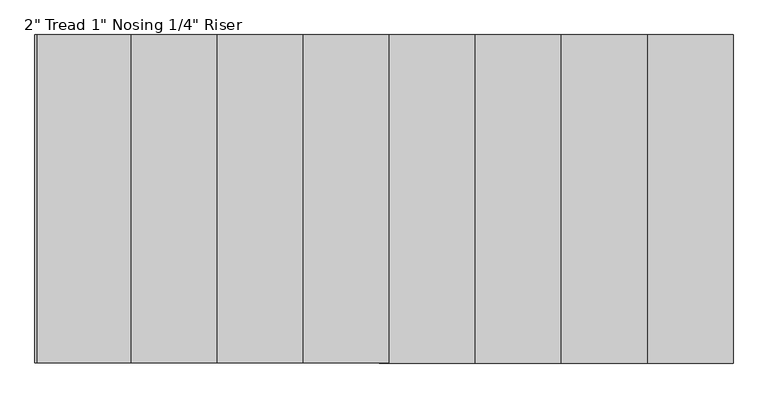
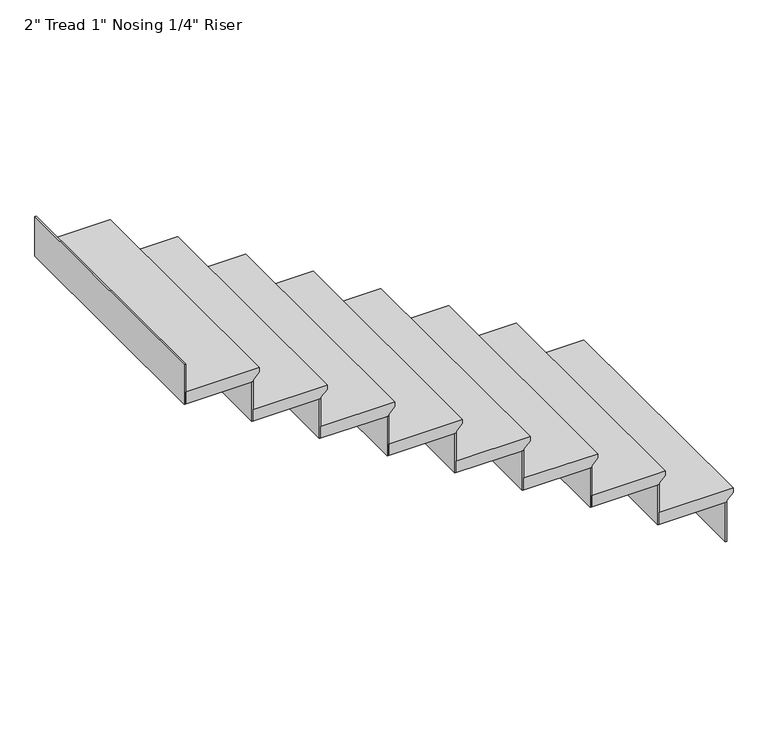
"""IFC4 building model written with IfcOpenShell, lengths in millimetres: stair flight geometry."""

from ifc_helpers import new_model, si_unit, origin, place, context, project, spatial, faceted_brep, source, transform, mapped, element, save


def stair_flight_205345c0(model_context):
    return source(origin(), model_context, "Body", "Brep", [
        faceted_brep([(665956.388677, -549416.0413841, 1710.8959459), (665956.388677, -549416.0413841, 1729.9459459), (665956.388677, -550482.8413841, 1729.9459459), (665956.388677, -550482.8413841, 1710.8959459), (665930.988677, -549416.0413841, 1685.4959459), (665930.988677, -550482.8413841, 1685.4959459), (665651.588677, -549416.0413841, 1729.9459459), (665651.588677, -550482.8413841, 1729.9459459), (665930.988677, -550482.8413841, 1679.1459459), (665651.588677, -550482.8413841, 1679.1459459), (665651.588677, -549416.0413841, 1679.1459459), (665930.988677, -549416.0413841, 1679.1459459)], [[[0, 1, 2, 3]], [[4, 0, 3, 5]], [[2, 1, 6, 7]], [[8, 9, 10, 11]], [[2, 7, 9, 8, 5, 3]], [[8, 11, 4, 5]], [[6, 1, 0, 4, 11, 10]], [[7, 6, 10, 9]]]),
        faceted_brep([(665930.988677, -549416.0413841, 1679.1459459), (665930.988677, -549416.0413841, 1506.1513514), (665924.638677, -549416.0413841, 1506.1513514), (665924.638677, -549416.0413841, 1679.1459459), (665930.988677, -550482.8413841, 1679.1459459), (665924.638677, -550482.8413841, 1679.1459459), (665924.638677, -550482.8413841, 1506.1513514), (665930.988677, -550482.8413841, 1506.1513514)], [[[0, 1, 2, 3]], [[4, 5, 6, 7]], [[1, 0, 4, 7]], [[2, 1, 7, 6]], [[3, 2, 6, 5]], [[0, 3, 5, 4]]]),
        faceted_brep([(665651.588677, -549416.0413841, 1852.1405405), (665651.588677, -549416.0413841, 1679.1459459), (665645.238677, -549416.0413841, 1679.1459459), (665645.238677, -549416.0413841, 1852.1405405), (665651.588677, -550482.8413841, 1852.1405405), (665645.238677, -550482.8413841, 1852.1405405), (665645.238677, -550482.8413841, 1679.1459459), (665651.588677, -550482.8413841, 1679.1459459)], [[[0, 1, 2, 3]], [[4, 5, 6, 7]], [[1, 0, 4, 7]], [[2, 1, 7, 6]], [[3, 2, 6, 5]], [[0, 3, 5, 4]]]),
        faceted_brep([(665676.988677, -550482.8413841, 1902.9405405), (665676.988677, -549416.0413841, 1902.9405405), (665372.188677, -549416.0413841, 1902.9405405), (665372.188677, -550482.8413841, 1902.9405405), (665651.588677, -550482.8413841, 1852.1405405), (665372.188677, -550482.8413841, 1852.1405405), (665372.188677, -549416.0413841, 1852.1405405), (665651.588677, -549416.0413841, 1852.1405405), (665651.588677, -550482.8413841, 1858.4905405), (665676.988677, -550482.8413841, 1883.8905405), (665651.588677, -549416.0413841, 1858.4905405), (665676.988677, -549416.0413841, 1883.8905405)], [[[0, 1, 2, 3]], [[4, 5, 6, 7]], [[0, 3, 5, 4, 8, 9]], [[4, 7, 10, 8]], [[2, 1, 11, 10, 7, 6]], [[3, 2, 6, 5]], [[11, 1, 0, 9]], [[10, 11, 9, 8]]]),
        faceted_brep([(665372.188677, -549416.0413841, 2025.1351351), (665372.188677, -549416.0413841, 1852.1405405), (665365.838677, -549416.0413841, 1852.1405405), (665365.838677, -549416.0413841, 2025.1351351), (665372.188677, -550482.8413841, 2025.1351351), (665365.838677, -550482.8413841, 2025.1351351), (665365.838677, -550482.8413841, 1852.1405405), (665372.188677, -550482.8413841, 1852.1405405)], [[[0, 1, 2, 3]], [[4, 5, 6, 7]], [[1, 0, 4, 7]], [[2, 1, 7, 6]], [[3, 2, 6, 5]], [[0, 3, 5, 4]]]),
        faceted_brep([(665397.588677, -550482.8413841, 2075.9351351), (665397.588677, -549416.0413841, 2075.9351351), (665092.788677, -549416.0413841, 2075.9351351), (665092.788677, -550482.8413841, 2075.9351351), (665372.188677, -550482.8413841, 2025.1351351), (665092.788677, -550482.8413841, 2025.1351351), (665092.788677, -549416.0413841, 2025.1351351), (665372.188677, -549416.0413841, 2025.1351351), (665372.188677, -550482.8413841, 2031.4851351), (665397.588677, -550482.8413841, 2056.8851351), (665372.188677, -549416.0413841, 2031.4851351), (665397.588677, -549416.0413841, 2056.8851351)], [[[0, 1, 2, 3]], [[4, 5, 6, 7]], [[0, 3, 5, 4, 8, 9]], [[4, 7, 10, 8]], [[2, 1, 11, 10, 7, 6]], [[3, 2, 6, 5]], [[11, 1, 0, 9]], [[10, 11, 9, 8]]]),
        faceted_brep([(665092.788677, -549416.0413841, 2198.1297297), (665092.788677, -549416.0413841, 2025.1351351), (665086.438677, -549416.0413841, 2025.1351351), (665086.438677, -549416.0413841, 2198.1297297), (665092.788677, -550482.8413841, 2198.1297297), (665086.438677, -550482.8413841, 2198.1297297), (665086.438677, -550482.8413841, 2025.1351351), (665092.788677, -550482.8413841, 2025.1351351)], [[[0, 1, 2, 3]], [[4, 5, 6, 7]], [[1, 0, 4, 7]], [[2, 1, 7, 6]], [[3, 2, 6, 5]], [[0, 3, 5, 4]]]),
        faceted_brep([(665118.188677, -550482.8413841, 2248.9297297), (665118.188677, -549416.0413841, 2248.9297297), (664813.388677, -549416.0413841, 2248.9297297), (664813.388677, -550482.8413841, 2248.9297297), (665092.788677, -550482.8413841, 2198.1297297), (664813.388677, -550482.8413841, 2198.1297297), (664813.388677, -549416.0413841, 2198.1297297), (665092.788677, -549416.0413841, 2198.1297297), (665092.788677, -550482.8413841, 2204.4797297), (665118.188677, -550482.8413841, 2229.8797297), (665092.788677, -549416.0413841, 2204.4797297), (665118.188677, -549416.0413841, 2229.8797297)], [[[0, 1, 2, 3]], [[4, 5, 6, 7]], [[0, 3, 5, 4, 8, 9]], [[4, 7, 10, 8]], [[2, 1, 11, 10, 7, 6]], [[3, 2, 6, 5]], [[11, 1, 0, 9]], [[10, 11, 9, 8]]]),
        faceted_brep([(664813.388677, -549416.0413841, 2371.1243243), (664813.388677, -549416.0413841, 2198.1297297), (664807.038677, -549416.0413841, 2198.1297297), (664807.038677, -549416.0413841, 2371.1243243), (664813.388677, -550482.8413841, 2371.1243243), (664807.038677, -550482.8413841, 2371.1243243), (664807.038677, -550482.8413841, 2198.1297297), (664813.388677, -550482.8413841, 2198.1297297)], [[[0, 1, 2, 3]], [[4, 5, 6, 7]], [[1, 0, 4, 7]], [[2, 1, 7, 6]], [[3, 2, 6, 5]], [[0, 3, 5, 4]]]),
        faceted_brep([(664838.788677, -550482.8413841, 2421.9243243), (664838.788677, -549416.0413841, 2421.9243243), (664533.988677, -549416.0413841, 2421.9243243), (664533.988677, -550482.8413841, 2421.9243243), (664813.388677, -550482.8413841, 2371.1243243), (664533.988677, -550482.8413841, 2371.1243243), (664533.988677, -549416.0413841, 2371.1243243), (664813.388677, -549416.0413841, 2371.1243243), (664813.388677, -550482.8413841, 2377.4743243), (664838.788677, -550482.8413841, 2402.8743243), (664813.388677, -549416.0413841, 2377.4743243), (664838.788677, -549416.0413841, 2402.8743243)], [[[0, 1, 2, 3]], [[4, 5, 6, 7]], [[0, 3, 5, 4, 8, 9]], [[4, 7, 10, 8]], [[2, 1, 11, 10, 7, 6]], [[3, 2, 6, 5]], [[11, 1, 0, 9]], [[10, 11, 9, 8]]]),
        faceted_brep([(664533.988677, -549416.0413841, 2544.1189189), (664533.988677, -549416.0413841, 2371.1243243), (664527.638677, -549416.0413841, 2371.1243243), (664527.638677, -549416.0413841, 2544.1189189), (664533.988677, -550482.8413841, 2544.1189189), (664527.638677, -550482.8413841, 2544.1189189), (664527.638677, -550482.8413841, 2371.1243243), (664533.988677, -550482.8413841, 2371.1243243)], [[[0, 1, 2, 3]], [[4, 5, 6, 7]], [[1, 0, 4, 7]], [[2, 1, 7, 6]], [[3, 2, 6, 5]], [[0, 3, 5, 4]]]),
        faceted_brep([(664559.388677, -550482.8413841, 2594.9189189), (664559.388677, -549416.0413841, 2594.9189189), (664254.588677, -549416.0413841, 2594.9189189), (664254.588677, -550482.8413841, 2594.9189189), (664533.988677, -550482.8413841, 2544.1189189), (664254.588677, -550482.8413841, 2544.1189189), (664254.588677, -549416.0413841, 2544.1189189), (664533.988677, -549416.0413841, 2544.1189189), (664533.988677, -550482.8413841, 2550.4689189), (664559.388677, -550482.8413841, 2575.8689189), (664533.988677, -549416.0413841, 2550.4689189), (664559.388677, -549416.0413841, 2575.8689189)], [[[0, 1, 2, 3]], [[4, 5, 6, 7]], [[0, 3, 5, 4, 8, 9]], [[4, 7, 10, 8]], [[2, 1, 11, 10, 7, 6]], [[3, 2, 6, 5]], [[11, 1, 0, 9]], [[10, 11, 9, 8]]]),
        faceted_brep([(664254.588677, -549416.0413841, 2717.1135135), (664254.588677, -549416.0413841, 2544.1189189), (664248.238677, -549416.0413841, 2544.1189189), (664248.238677, -549416.0413841, 2717.1135135), (664254.588677, -550482.8413841, 2717.1135135), (664248.238677, -550482.8413841, 2717.1135135), (664248.238677, -550482.8413841, 2544.1189189), (664254.588677, -550482.8413841, 2544.1189189)], [[[0, 1, 2, 3]], [[4, 5, 6, 7]], [[1, 0, 4, 7]], [[2, 1, 7, 6]], [[3, 2, 6, 5]], [[0, 3, 5, 4]]]),
        faceted_brep([(664279.988677, -550482.8413841, 2767.9135135), (664279.988677, -549416.0413841, 2767.9135135), (663975.188677, -549416.0413841, 2767.9135135), (663975.188677, -550482.8413841, 2767.9135135), (664254.588677, -550482.8413841, 2717.1135135), (663975.188677, -550482.8413841, 2717.1135135), (663975.188677, -549416.0413841, 2717.1135135), (664254.588677, -549416.0413841, 2717.1135135), (664254.588677, -550482.8413841, 2723.4635135), (664279.988677, -550482.8413841, 2748.8635135), (664254.588677, -549416.0413841, 2723.4635135), (664279.988677, -549416.0413841, 2748.8635135)], [[[0, 1, 2, 3]], [[4, 5, 6, 7]], [[0, 3, 5, 4, 8, 9]], [[4, 7, 10, 8]], [[2, 1, 11, 10, 7, 6]], [[3, 2, 6, 5]], [[11, 1, 0, 9]], [[10, 11, 9, 8]]]),
        faceted_brep([(663695.788677, -549416.0413841, 3063.1027027), (663695.788677, -549416.0413841, 2890.1081081), (663689.438677, -549416.0413841, 2890.1081081), (663689.438677, -549416.0413841, 3063.1027027), (663695.788677, -550482.8413841, 3063.1027027), (663689.438677, -550482.8413841, 3063.1027027), (663689.438677, -550482.8413841, 2890.1081081), (663695.788677, -550482.8413841, 2890.1081081)], [[[0, 1, 2, 3]], [[4, 5, 6, 7]], [[1, 0, 4, 7]], [[2, 1, 7, 6]], [[3, 2, 6, 5]], [[0, 3, 5, 4]]]),
        faceted_brep([(663975.188677, -549416.0413841, 2890.1081081), (663975.188677, -549416.0413841, 2717.1135135), (663968.838677, -549416.0413841, 2717.1135135), (663968.838677, -549416.0413841, 2890.1081081), (663975.188677, -550482.8413841, 2890.1081081), (663968.838677, -550482.8413841, 2890.1081081), (663968.838677, -550482.8413841, 2717.1135135), (663975.188677, -550482.8413841, 2717.1135135)], [[[0, 1, 2, 3]], [[4, 5, 6, 7]], [[1, 0, 4, 7]], [[2, 1, 7, 6]], [[3, 2, 6, 5]], [[0, 3, 5, 4]]]),
        faceted_brep([(664000.588677, -550482.8413841, 2940.9081081), (664000.588677, -549416.0413841, 2940.9081081), (663721.188677, -549416.0413841, 2940.9081081), (663695.788677, -549416.0413841, 2940.9081081), (663695.788677, -550482.8413841, 2940.9081081), (663975.188677, -550482.8413841, 2890.1081081), (663695.788677, -550482.8413841, 2890.1081081), (663695.788677, -549416.0413841, 2890.1081081), (663721.188677, -549416.0413841, 2890.1081081), (663975.188677, -549416.0413841, 2890.1081081), (663975.188677, -550482.8413841, 2896.4581081), (664000.588677, -550482.8413841, 2921.8581081), (663975.188677, -549416.0413841, 2896.4581081), (664000.588677, -549416.0413841, 2921.8581081)], [[[0, 1, 2, 3, 4]], [[5, 6, 7, 8, 9]], [[0, 4, 6, 5, 10, 11]], [[5, 9, 12, 10]], [[2, 1, 13, 12, 9, 8]], [[3, 2, 8, 7]], [[4, 3, 7, 6]], [[13, 1, 0, 11]], [[12, 13, 11, 10]]]),
    ])


if __name__ == "__main__":
    model = new_model("IFC4")
    model_context = context("Model", 3, world=origin())
    ifc_project = project(units=[si_unit("LENGTHUNIT", "METRE", prefix="MILLI")], contexts=[model_context])
    site = spatial("IfcSite", under=ifc_project)
    building = spatial("IfcBuilding", under=site)
    placement = place(None, origin())
    stair_flight_shape = stair_flight_205345c0(model_context)
    element("IfcStairFlight", 1, ObjectType="2\" Tread 1\" Nosing 1/4\" Riser", at=placement, inside=building, context=model_context, shape_type="MappedRepresentation", body=[
        mapped(stair_flight_shape, transform((0.0, 0.0, 0.0), x_axis=(1.0, 0.0, 0.0), y_axis=(0.0, 1.0, 0.0), z_axis=(0.0, 0.0, 1.0))),
    ])
    save(model, "model.ifc")
